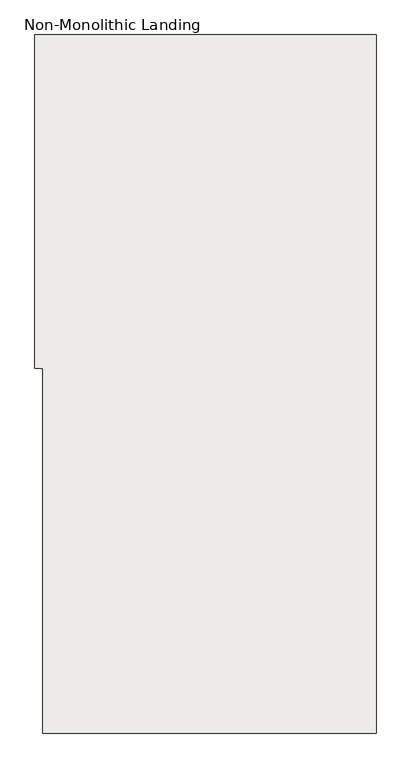
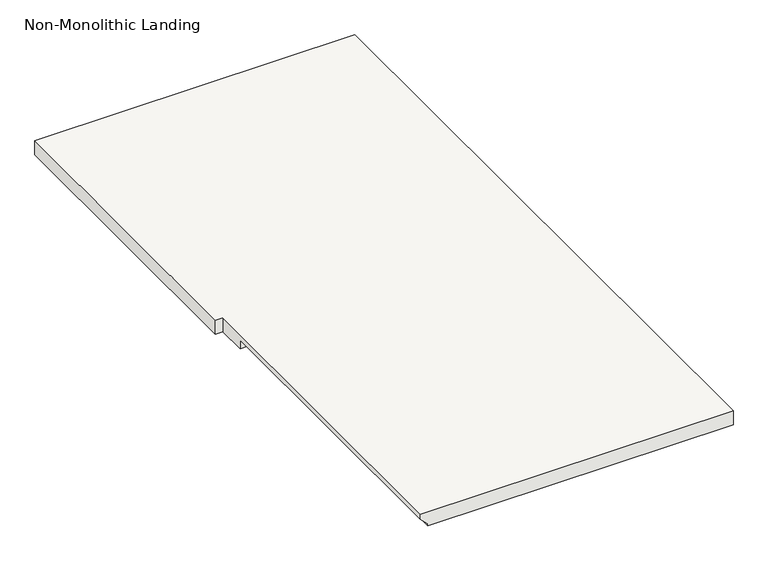
"""IFC4 building model written with IfcOpenShell, lengths in millimetres: slab geometry, Non-Monolithic Landing."""

from ifc_helpers import new_model, si_unit, origin, place, context, project, spatial, faceted_brep, source, transform, mapped, element, save


def non_monolithic_landing_a18c07da(model_context):
    return source(origin(), model_context, "Body", "Brep", [
        faceted_brep([(665981.788677, -551651.2413841, 1067.6581081), (665956.388677, -551651.2413841, 1093.0581081), (665956.388677, -550584.4413841, 1093.0581081), (665981.788677, -550584.4413841, 1067.6581081), (667023.188677, -551651.2413841, 1112.1081081), (667023.188677, -549416.0413841, 1112.1081081), (665956.388677, -549416.0413841, 1112.1081081), (665930.988677, -549416.0413841, 1112.1081081), (665930.988677, -550482.8413841, 1112.1081081), (665956.388677, -550482.8413841, 1112.1081081), (665956.388677, -551651.2413841, 1112.1081081), (665981.788677, -550584.4413841, 1061.3081081), (665956.388677, -550584.4413841, 1061.3081081), (665956.388677, -550482.8413841, 1061.3081081), (665930.988677, -550482.8413841, 1061.3081081), (665930.988677, -549416.0413841, 1061.3081081), (665956.388677, -549416.0413841, 1061.3081081), (667023.188677, -549416.0413841, 1061.3081081), (667023.188677, -551651.2413841, 1061.3081081), (665981.788677, -551651.2413841, 1061.3081081)], [[[0, 1, 2, 3]], [[4, 5, 6, 7, 8, 9, 10]], [[11, 12, 13, 14, 15, 16, 17, 18, 19]], [[12, 11, 3, 2]], [[11, 19, 0, 3]], [[4, 10, 1, 0, 19, 18]], [[5, 4, 18, 17]], [[6, 5, 17, 16]], [[7, 6, 16, 15]], [[8, 7, 15, 14]], [[9, 8, 14, 13]], [[10, 9, 13, 12, 2, 1]]]),
    ])


if __name__ == "__main__":
    model = new_model("IFC4")
    model_context = context("Model", 3, world=origin())
    ifc_project = project(units=[si_unit("LENGTHUNIT", "METRE", prefix="MILLI")], contexts=[model_context])
    site = spatial("IfcSite", under=ifc_project)
    building = spatial("IfcBuilding", under=site)
    placement = place(None, origin())
    non_monolithic_landing_shape = non_monolithic_landing_a18c07da(model_context)
    element("IfcSlab", 1, ObjectType="Non-Monolithic Landing", at=placement, inside=building, context=model_context, shape_type="MappedRepresentation", body=[
        mapped(non_monolithic_landing_shape, transform((0.0, 0.0, 0.0), x_axis=(1.0, 0.0, 0.0), y_axis=(0.0, 1.0, 0.0), z_axis=(0.0, 0.0, 1.0))),
    ])
    save(model, "model.ifc")
